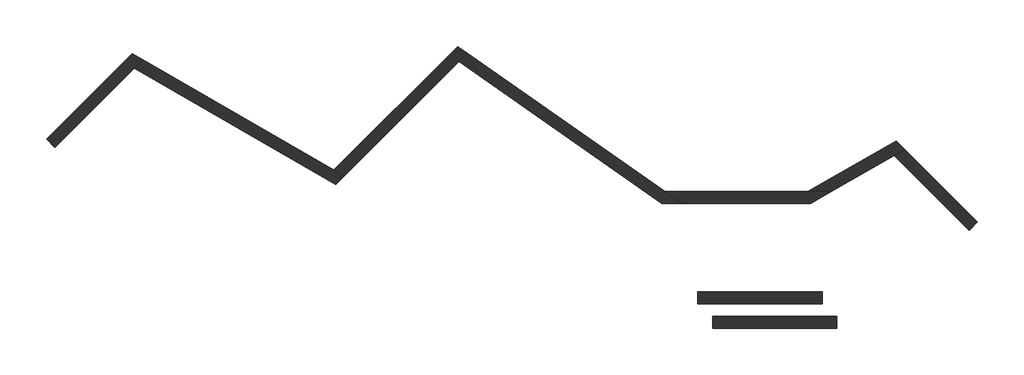
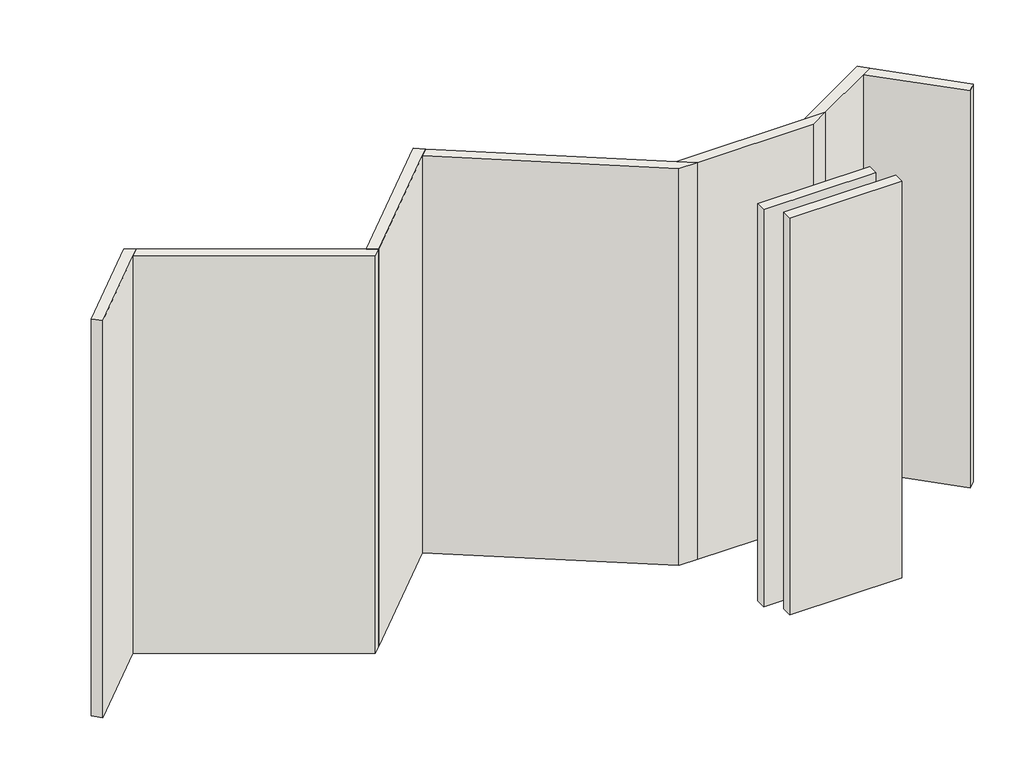
# One storey: 9 walls.
"""IFC4 building model written with IfcOpenShell, lengths in millimetres."""

import ifcopenshell
import ifcopenshell.guid

model = None  # the IFC model being written
_history = None  # IfcOwnerHistory: only IFC2X3 demands one
_inside = {}  # id of a spatial element -> (the spatial element, [elements in it])
_under = {}  # id of a project, library or spatial element -> (it, [spatial elements below it])
_declared = {}  # id of a project -> (the project, [libraries it declares])
_typed = {}  # id of a type object -> (the type object, [elements of that type])
_made_of = {}  # id of a material, layer set ... -> (it, [elements and type objects made of it])


def new_model(schema):
    """Start an empty IFC model of exactly this schema.

    Asked for "IFC4X3", IfcOpenShell would pick the latest addendum, in which some entities
    have other attributes; the version numbers below select the first issue.
    IFC2X3 requires an IfcOwnerHistory on every rooted entity: one is made here for all.
    """
    global model, _history
    if schema == "IFC4X3":
        model = ifcopenshell.file(schema_version=(4, 3, 0, 0))
    else:
        model = ifcopenshell.file(schema=schema)
    _inside.clear()
    _under.clear()
    _declared.clear()
    _typed.clear()
    _made_of.clear()
    _history = None
    if model.schema == "IFC2X3":
        org = make("IfcOrganization", Name="unknown")
        user = make(
            "IfcPersonAndOrganization",
            ThePerson=make("IfcPerson", FamilyName="unknown"),
            TheOrganization=org,
        )
        app = make(
            "IfcApplication",
            ApplicationDeveloper=org,
            Version="unknown",
            ApplicationFullName="unknown",
            ApplicationIdentifier="unknown",
        )
        _history = make(
            "IfcOwnerHistory",
            OwningUser=user,
            OwningApplication=app,
            ChangeAction="ADDED",
            CreationDate=0,
        )
    return model


def make(cls, **values):
    """One entity of the class cls with the attributes given. An attribute that is None is left unset."""
    return model.create_entity(
        cls, **{name: value for name, value in values.items() if value is not None}
    )


def rooted(cls, **values):
    """An entity with a GlobalId (a new one), such as an element, a storey or a relation."""
    return make(cls, GlobalId=ifcopenshell.guid.new(), OwnerHistory=_history, **values)


def si_unit(unit_type, name, prefix=None):
    """IfcSIUnit, for example si_unit("LENGTHUNIT", "METRE", prefix="MILLI")."""
    return make("IfcSIUnit", UnitType=unit_type, Prefix=prefix, Name=name)


def assignment(units):
    """IfcUnitAssignment: the units of a project."""
    return None if units is None else make("IfcUnitAssignment", Units=units)


def point(xyz):
    """IfcCartesianPoint."""
    return None if xyz is None else make("IfcCartesianPoint", Coordinates=xyz)


def direction(xyz):
    """IfcDirection."""
    return None if xyz is None else make("IfcDirection", DirectionRatios=xyz)


def frame(location, z_axis=None, x_axis=None):
    """IfcAxis2Placement3D, a coordinate frame: its origin and axes. An axis left out is left unset."""
    return make(
        "IfcAxis2Placement3D",
        Location=point(location),
        Axis=direction(z_axis),
        RefDirection=direction(x_axis),
    )


def origin():
    """The frame at (0, 0, 0) with its axes left unset."""
    return frame((0.0, 0.0, 0.0))


def origin_with_axes():
    """The frame at (0, 0, 0) with the z axis (0, 0, 1) and the x axis (1, 0, 0) written out."""
    return frame((0.0, 0.0, 0.0), z_axis=(0.0, 0.0, 1.0), x_axis=(1.0, 0.0, 0.0))


def place(relative_to, where):
    """IfcLocalPlacement: puts the frame where relative to a parent placement (None: the world)."""
    return make(
        "IfcLocalPlacement", PlacementRelTo=relative_to, RelativePlacement=where
    )


def context(
    kind, dimensions, precision=None, world=None, true_north=None, identifier=None
):
    """IfcGeometricRepresentationContext, for example the 3D "Model" context."""
    return make(
        "IfcGeometricRepresentationContext",
        ContextIdentifier=identifier,
        ContextType=kind,
        CoordinateSpaceDimension=dimensions,
        Precision=precision,
        WorldCoordinateSystem=world,
        TrueNorth=true_north,
    )


def project(units=None, contexts=None):
    """IfcProject with its units and contexts."""
    return rooted(
        "IfcProject",
        Name="project",
        RepresentationContexts=contexts,
        UnitsInContext=assignment(units),
    )


def spatial(cls, under=None, at=None, **own):
    """A site, building, storey or space (cls), placed at a placement, below another one or the project."""
    s = rooted(cls, ObjectPlacement=at, **own)
    if under is not None:
        _under.setdefault(under.id(), (under, []))[1].append(s)
    return s


def polyline(points):
    """IfcPolyline through the points."""
    return make("IfcPolyline", Points=[point(p) for p in points])


def outline(outer, holes=None, kind="AREA"):
    """IfcArbitraryClosedProfileDef: a profile drawn as a closed curve; with holes, ...WithVoids."""
    if holes is None:
        return make("IfcArbitraryClosedProfileDef", ProfileType=kind, OuterCurve=outer)
    return make(
        "IfcArbitraryProfileDefWithVoids",
        ProfileType=kind,
        OuterCurve=outer,
        InnerCurves=holes,
    )


def extrude(swept, where, along, depth):
    """IfcExtrudedAreaSolid: the profile swept, set in the frame where, extruded along a direction by depth."""
    return make(
        "IfcExtrudedAreaSolid",
        SweptArea=swept,
        Position=where,
        ExtrudedDirection=direction(along),
        Depth=depth,
    )


def faces_of(points, faces, orient=None, outer=None):
    """IfcFace entities. A face is a list of loops; a loop is a list of indices into points, from 0.

    orient and outer hold one flag for each loop. By default every Orientation is true, the
    first loop of a face is its IfcFaceOuterBound and the others are IfcFaceBound.
    """
    made = []
    for i, loops in enumerate(faces):
        bounds = []
        for j, loop in enumerate(loops):
            is_outer = j == 0 if outer is None else outer[i][j]
            bounds.append(
                make(
                    "IfcFaceOuterBound" if is_outer else "IfcFaceBound",
                    Bound=make("IfcPolyLoop", Polygon=[points[k] for k in loop]),
                    Orientation=True if orient is None else orient[i][j],
                )
            )
        made.append(make("IfcFace", Bounds=bounds))
    return made


def faceted_brep(points, faces, orient=None, outer=None, voids=None):
    """IfcFacetedBrep: a solid bounded by flat faces; with voids (closed shells), ...WithVoids."""
    shared = [point(p) for p in points]
    hull = make("IfcClosedShell", CfsFaces=faces_of(shared, faces, orient, outer))
    if voids is None:
        return make("IfcFacetedBrep", Outer=hull)
    return make(
        "IfcFacetedBrepWithVoids",
        Outer=hull,
        Voids=[
            make(cls, CfsFaces=faces_of(shared, fs, o, b)) for cls, fs, o, b in voids
        ],
    )


def shape(context_of_items, identifier, shape_type, items):
    """IfcShapeRepresentation: the items that make up one representation, for example the "Body"."""
    return make(
        "IfcShapeRepresentation",
        ContextOfItems=context_of_items,
        RepresentationIdentifier=identifier,
        RepresentationType=shape_type,
        Items=items,
    )


def made_of(thing, what):
    """Note that an element or type object is made of a material, layer set ...; save() writes the relation."""
    if what is not None:
        _made_of.setdefault(what.id(), (what, []))[1].append(thing)
    return thing


def element(
    cls,
    number,
    at=None,
    inside=None,
    cuts=None,
    type_object=None,
    material=None,
    context=None,
    identifier="Body",
    shape_type=None,
    held_by="IfcProductDefinitionShape",
    body=None,
    shapes=None,
    **own,
):
    """One element of the class cls, such as IfcWall. Its Tag is "e" and its number.

    at: its placement. inside: the storey or other place that contains it. cuts: it is an
    opening in that element (IfcRelVoidsElement). A single representation is given by context,
    identifier, shape_type and body (its items); several are given by shapes. held_by: the class
    of the entity that holds the representations. save() writes the other relations.
    """
    e = rooted(cls, Tag="e%d" % number, ObjectPlacement=at, **own)
    if body is not None:
        shapes = [shape(context, identifier, shape_type, body)]
    if shapes is not None:
        e.Representation = make(held_by, Representations=shapes)
    if inside is not None:
        _inside.setdefault(inside.id(), (inside, []))[1].append(e)
    if cuts is not None:
        rooted(
            "IfcRelVoidsElement", RelatingBuildingElement=cuts, RelatedOpeningElement=e
        )
    if type_object is not None:
        _typed.setdefault(type_object.id(), (type_object, []))[1].append(e)
    return made_of(e, material)


def aggregate(whole, parts):
    """IfcRelAggregates: a whole, such as a stair, and the parts it consists of."""
    return rooted("IfcRelAggregates", RelatingObject=whole, RelatedObjects=parts)


def save(model, path):
    """Write the relations noted so far, then the file.

    IfcRelAggregates (storeys below a building ...), IfcRelContainedInSpatialStructure (elements
    in a storey), IfcRelDefinesByType, IfcRelAssociatesMaterial and IfcRelDeclares: one each for
    every whole, place, type object, material and project.
    """
    for whole, parts in _under.values():
        aggregate(whole, parts)
    for where, things in _inside.values():
        rooted(
            "IfcRelContainedInSpatialStructure",
            RelatedElements=things,
            RelatingStructure=where,
        )
    for kind, things in _typed.values():
        rooted("IfcRelDefinesByType", RelatedObjects=things, RelatingType=kind)
    for what, things in _made_of.values():
        rooted("IfcRelAssociatesMaterial", RelatedObjects=things, RelatingMaterial=what)
    for by, libraries in _declared.values():
        rooted("IfcRelDeclares", RelatingContext=by, RelatedDefinitions=libraries)
    model.write(path)


model = new_model("IFC4")

# Units and contexts
model_context = context("Model", 3, world=origin())
ifc_project = project(units=[si_unit("LENGTHUNIT", "METRE", prefix="MILLI")], contexts=[model_context])

# Site, building, storey
site = spatial("IfcSite", under=ifc_project)
building = spatial("IfcBuilding", under=site)
storey = spatial("IfcBuildingStorey", under=building, Name="Уровень 1", Elevation=0.0)

# Walls
placement = place(None, origin())
element("IfcWall", 1, ObjectType="Типовой - 200мм", at=placement, inside=storey, context=model_context, shape_type="Brep", body=[
    faceted_brep([(-11036.9996374, 2584.0231166, 0.0), (-9677.0442867, 3943.9784673, 0.0), (-9530.6341252, 4090.3886288, 0.0), (-9530.6341252, 4090.3886288, 8000.0), (-9677.0442867, 3943.9784673, 8000.0), (-11036.9996374, 2584.0231166, 8000.0), (-11178.4209937, 2725.4444728, 0.0), (-11178.4209937, 2725.4444728, 8000.0), (-9709.9492196, 4193.9162469, 8000.0), (-9709.9492196, 4193.9162469, 0.0)], [[[0, 1, 2, 3, 4, 5]], [[6, 7, 8, 9]], [[2, 1, 0, 6, 9]], [[5, 4, 3, 8, 7]], [[0, 5, 7, 6]], [[3, 2, 9, 8]]]),
])
element("IfcWall", 2, ObjectType="Типовой - 200мм", at=placement, inside=storey, context=model_context, shape_type="Brep", body=[
    faceted_brep([(-9677.0442867, 3943.9784673, 0.0), (-6212.9426716, 1943.9784673, 0.0), (-6212.9426716, 1943.9784673, 8000.0), (-9677.0442867, 3943.9784673, 8000.0), (-9530.6341252, 4090.3886288, 0.0), (-9530.6341252, 4090.3886288, 8000.0), (-6245.8476045, 2193.9162469, 8000.0), (-6066.5325101, 2090.3886288, 8000.0), (-6066.5325101, 2090.3886288, 0.0), (-6245.8476045, 2193.9162469, 0.0)], [[[0, 1, 2, 3]], [[4, 5, 6, 7, 8, 9]], [[1, 0, 4, 9, 8]], [[3, 2, 7, 6, 5]], [[0, 3, 5, 4]], [[2, 1, 8, 7]]]),
])
element("IfcWall", 3, ObjectType="Типовой - 200мм", at=placement, inside=storey, context=model_context, shape_type="Brep", body=[
    faceted_brep([(-6066.5325101, 2090.3886288, 0.0), (-4096.6974203, 4060.2237186, 0.0), (-3953.0944117, 4203.8267272, 0.0), (-3953.0944117, 4203.8267272, 8000.0), (-4096.6974203, 4060.2237186, 8000.0), (-6066.5325101, 2090.3886288, 8000.0), (-6245.8476045, 2193.9162469, 0.0), (-6245.8476045, 2193.9162469, 8000.0), (-4119.4521687, 4320.3116827, 8000.0), (-4119.4521687, 4320.3116827, 0.0)], [[[0, 1, 2, 3, 4, 5]], [[6, 7, 8, 9]], [[2, 1, 0, 6, 9]], [[5, 4, 3, 8, 7]], [[0, 5, 7, 6]], [[3, 2, 9, 8]]]),
])
element("IfcWall", 4, ObjectType="Типовой - 200мм", at=placement, inside=storey, context=model_context, shape_type="Brep", body=[
    faceted_brep([(-4096.6974203, 4060.2237186, 0.0), (-617.2508829, 1623.8890243, 0.0), (-617.2508829, 1623.8890243, 8000.0), (-4096.6974203, 4060.2237186, 8000.0), (-3953.0944117, 4203.8267272, 0.0), (-3953.0944117, 4203.8267272, 8000.0), (-554.1911251, 1823.8890243, 8000.0), (-268.5615238, 1623.8890243, 8000.0), (-268.5615238, 1623.8890243, 0.0), (-554.1911251, 1823.8890243, 0.0)], [[[0, 1, 2, 3]], [[4, 5, 6, 7, 8, 9]], [[1, 0, 4, 9, 8]], [[3, 2, 7, 6, 5]], [[0, 3, 5, 4]], [[2, 1, 8, 7]]]),
])
element("IfcWall", 5, ObjectType="Типовой - 200мм", at=placement, inside=storey, context=model_context, shape_type="Brep", body=[
    faceted_brep([(-268.5615238, 1623.8890243, 0.0), (1941.0739152, 1623.8890243, 0.0), (1941.0739152, 1623.8890243, 8000.0), (-268.5615238, 1623.8890243, 8000.0), (-554.1911251, 1823.8890243, 0.0), (-554.1911251, 1823.8890243, 8000.0), (1887.4840767, 1823.8890243, 8000.0), (2287.4840767, 1823.8890243, 8000.0), (2287.4840767, 1823.8890243, 0.0), (1887.4840767, 1823.8890243, 0.0)], [[[0, 1, 2, 3]], [[4, 5, 6, 7, 8, 9]], [[1, 0, 4, 9, 8]], [[3, 2, 7, 6, 5]], [[0, 3, 5, 4]], [[2, 1, 8, 7]]]),
])
element("IfcWall", 6, ObjectType="Типовой - 200мм", at=placement, inside=storey, context=model_context, shape_type="Brep", body=[
    faceted_brep([(2287.4840767, 1823.8890243, 0.0), (3370.0697159, 2448.9201346, 0.0), (3549.3848104, 2552.4477526, 0.0), (3549.3848104, 2552.4477526, 8000.0), (3370.0697159, 2448.9201346, 8000.0), (2287.4840767, 1823.8890243, 8000.0), (1887.4840767, 1823.8890243, 0.0), (1887.4840767, 1823.8890243, 8000.0), (3402.9746489, 2698.8579141, 8000.0), (3402.9746489, 2698.8579141, 0.0)], [[[0, 1, 2, 3, 4, 5]], [[6, 7, 8, 9]], [[2, 1, 0, 6, 9]], [[5, 4, 3, 8, 7]], [[0, 5, 7, 6]], [[3, 2, 9, 8]]]),
])
element("IfcWall", 7, ObjectType="Типовой - 200мм", at=placement, inside=storey, context=model_context, shape_type="SweptSolid", body=[
    extrude(outline(polyline([(4659.3143885, 1159.675462), (3370.0697159, 2448.9201346), (3549.3848104, 2552.4477526), (4800.7357448, 1301.0968182), (4659.3143885, 1159.675462)])), origin_with_axes(), (0.0, 0.0, 1.0), 8000.0),
])
element("IfcWall", 8, ObjectType="Типовой - 200мм", at=placement, inside=storey, context=model_context, shape_type="SweptSolid", body=[
    extrude(outline(polyline([(2133.6, -100.0), (0.0, -100.0), (0.0, 100.0), (2133.6, 100.0), (2133.6, -100.0)])), origin_with_axes(), (0.0, 0.0, 1.0), 8000.0),
])
element("IfcWall", 9, ObjectType="Типовой - 200мм", at=placement, inside=storey, context=model_context, shape_type="SweptSolid", body=[
    extrude(outline(polyline([(2387.6, -521.3468146), (254.0, -521.3468146), (254.0, -321.3468146), (2387.6, -321.3468146), (2387.6, -521.3468146)])), origin_with_axes(), (0.0, 0.0, 1.0), 8000.0),
])

save(model, "model.ifc")

# Revit data of these elements
# Project information
#   Дата утверждения проекта = "Дата выпуска"
#   Статус проекта = "Статус проекта"
#   Заказчик = "Владелец"
#   Адрес проекта = "Укажите адрес"
#   Наименование проекта = "Наименование проекта"
#   Номер проекта = "0001"
# Type "Типовой - 200мм"
#   Type Mark = "qwe qwe"
#   Layers, outside or top first: 0.656167979 ft no material (function 1)
# Elements 1, 2, 3, 4, 5, 6, 7, 8, 9 (IfcWall, "Типовой - 200мм")
#   Top Offset = 0.000000000 ft
#   Base Offset = 0.000000000 ft
#   Unconnected Height = 26.246719160 ft
#   wall height = 26.246719160 ft
#   Phase Created = Стадия 1
#   Base Constraint = Уровень 1
#   Materials on its faces: "Стена по умолчанию"
# Materials
#   "Стена по умолчанию": class "Разное", colour RGB 128 128 128, transparency 0, Cost = 0
